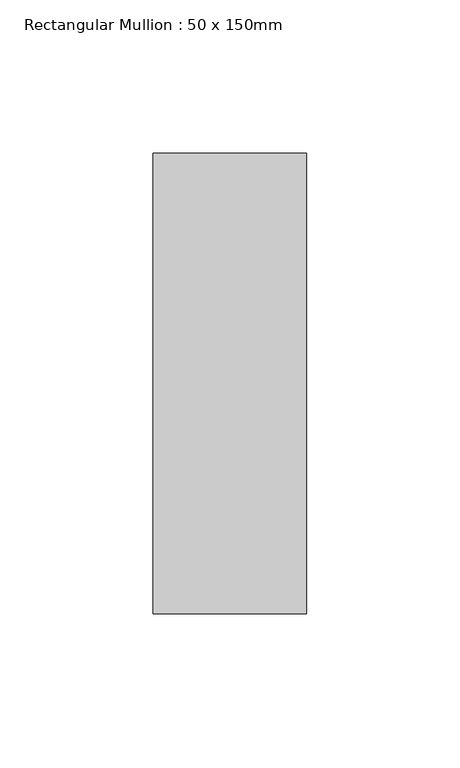
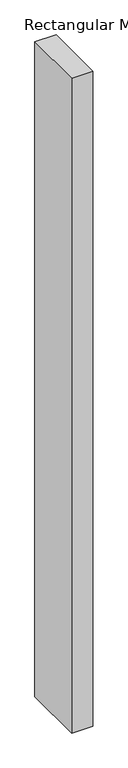
"""IFC4 building model written with IfcOpenShell, lengths in millimetres: member geometry, Rectangular Mullion : 50 x 150mm."""

from ifc_helpers import new_model, si_unit, frame, origin, place, context, project, spatial, polyline, outline, extrude, source, transform, mapped, element, save


def rectangular_mullion_50_x_150mm_a5738571(model_context):
    return source(origin(), model_context, "Body", "SweptSolid", [
        extrude(outline(polyline([(0.0, 75.0), (0.0, -75.0), (-50.0, -75.0), (-50.0, 75.0), (0.0, 75.0)])), frame((0.0, 0.0, -1635.0991456), z_axis=(0.0, 0.0, 1.0), x_axis=(1.0, 0.0, 0.0)), (0.0, 0.0, 1.0), 1635.0991456),
    ])


if __name__ == "__main__":
    model = new_model("IFC4")
    model_context = context("Model", 3, world=origin())
    ifc_project = project(units=[si_unit("LENGTHUNIT", "METRE", prefix="MILLI")], contexts=[model_context])
    site = spatial("IfcSite", under=ifc_project)
    building = spatial("IfcBuilding", under=site)
    placement = place(None, origin())
    rectangular_mullion_50_x_150mm_shape = rectangular_mullion_50_x_150mm_a5738571(model_context)
    element("IfcMember", 1, ObjectType="Rectangular Mullion : 50 x 150mm", at=placement, inside=building, context=model_context, shape_type="MappedRepresentation", body=[
        mapped(rectangular_mullion_50_x_150mm_shape, transform((0.0, 0.0, 0.0), x_axis=(1.0, 0.0, 0.0), y_axis=(0.0, 1.0, 0.0), z_axis=(0.0, 0.0, 1.0))),
    ])
    save(model, "model.ifc")

# Revit data of these elements
# Type "Rectangular Mullion : 50 x 150mm"
#   built-in parameter 1007304 = 0.492126 (stored number, unit not read)
#   built-in parameter 1007301 = 0.082021 (stored number, unit not read)
#   built-in parameter 1007300 = 0.082021 (stored number, unit not read)
# Element 1 (IfcMember, "Rectangular Mullion : 50 x 150mm")
#   Materials on its faces: "Aluminium"
# Materials
#   "Aluminium": class "Metal", colour RGB 247 247 247, transparency 0, Description = "Aluminium 6061", Cost = 0
